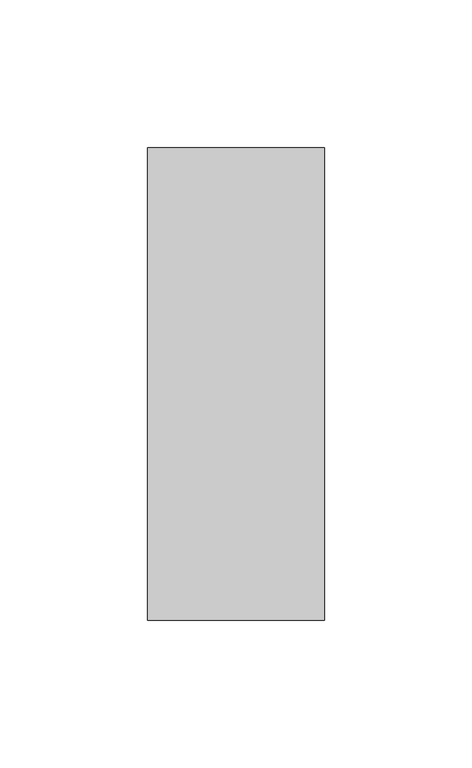
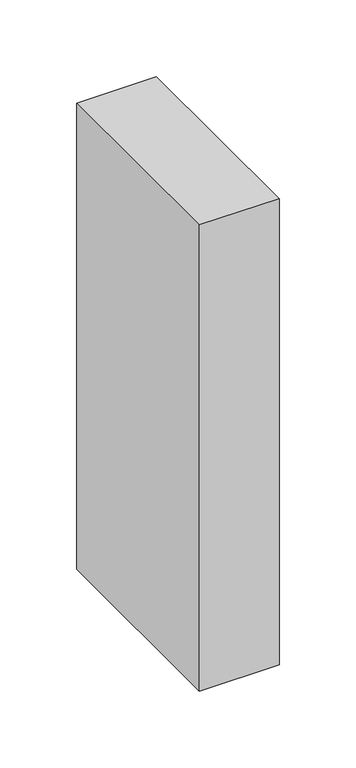
"""IFC4 building model written with IfcOpenShell, lengths in millimetres: column geometry, Madeira de lei-Coluna : Pontalete 6X16cm."""

import ifcopenshell
import ifcopenshell.guid

model = None  # the IFC model being written
_history = None  # IfcOwnerHistory: only IFC2X3 demands one
_inside = {}  # id of a spatial element -> (the spatial element, [elements in it])
_under = {}  # id of a project, library or spatial element -> (it, [spatial elements below it])
_declared = {}  # id of a project -> (the project, [libraries it declares])
_typed = {}  # id of a type object -> (the type object, [elements of that type])
_made_of = {}  # id of a material, layer set ... -> (it, [elements and type objects made of it])


def new_model(schema):
    """Start an empty IFC model of exactly this schema.

    Asked for "IFC4X3", IfcOpenShell would pick the latest addendum, in which some entities
    have other attributes; the version numbers below select the first issue.
    IFC2X3 requires an IfcOwnerHistory on every rooted entity: one is made here for all.
    """
    global model, _history
    if schema == "IFC4X3":
        model = ifcopenshell.file(schema_version=(4, 3, 0, 0))
    else:
        model = ifcopenshell.file(schema=schema)
    _inside.clear()
    _under.clear()
    _declared.clear()
    _typed.clear()
    _made_of.clear()
    _history = None
    if model.schema == "IFC2X3":
        org = make("IfcOrganization", Name="unknown")
        user = make(
            "IfcPersonAndOrganization",
            ThePerson=make("IfcPerson", FamilyName="unknown"),
            TheOrganization=org,
        )
        app = make(
            "IfcApplication",
            ApplicationDeveloper=org,
            Version="unknown",
            ApplicationFullName="unknown",
            ApplicationIdentifier="unknown",
        )
        _history = make(
            "IfcOwnerHistory",
            OwningUser=user,
            OwningApplication=app,
            ChangeAction="ADDED",
            CreationDate=0,
        )
    return model


def make(cls, **values):
    """One entity of the class cls with the attributes given. An attribute that is None is left unset."""
    return model.create_entity(
        cls, **{name: value for name, value in values.items() if value is not None}
    )


def rooted(cls, **values):
    """An entity with a GlobalId (a new one), such as an element, a storey or a relation."""
    return make(cls, GlobalId=ifcopenshell.guid.new(), OwnerHistory=_history, **values)


def si_unit(unit_type, name, prefix=None):
    """IfcSIUnit, for example si_unit("LENGTHUNIT", "METRE", prefix="MILLI")."""
    return make("IfcSIUnit", UnitType=unit_type, Prefix=prefix, Name=name)


def assignment(units):
    """IfcUnitAssignment: the units of a project."""
    return None if units is None else make("IfcUnitAssignment", Units=units)


def point(xyz):
    """IfcCartesianPoint."""
    return None if xyz is None else make("IfcCartesianPoint", Coordinates=xyz)


def direction(xyz):
    """IfcDirection."""
    return None if xyz is None else make("IfcDirection", DirectionRatios=xyz)


def frame(location, z_axis=None, x_axis=None):
    """IfcAxis2Placement3D, a coordinate frame: its origin and axes. An axis left out is left unset."""
    return make(
        "IfcAxis2Placement3D",
        Location=point(location),
        Axis=direction(z_axis),
        RefDirection=direction(x_axis),
    )


def origin():
    """The frame at (0, 0, 0) with its axes left unset."""
    return frame((0.0, 0.0, 0.0))


def place(relative_to, where):
    """IfcLocalPlacement: puts the frame where relative to a parent placement (None: the world)."""
    return make(
        "IfcLocalPlacement", PlacementRelTo=relative_to, RelativePlacement=where
    )


def context(
    kind, dimensions, precision=None, world=None, true_north=None, identifier=None
):
    """IfcGeometricRepresentationContext, for example the 3D "Model" context."""
    return make(
        "IfcGeometricRepresentationContext",
        ContextIdentifier=identifier,
        ContextType=kind,
        CoordinateSpaceDimension=dimensions,
        Precision=precision,
        WorldCoordinateSystem=world,
        TrueNorth=true_north,
    )


def project(units=None, contexts=None):
    """IfcProject with its units and contexts."""
    return rooted(
        "IfcProject",
        Name="project",
        RepresentationContexts=contexts,
        UnitsInContext=assignment(units),
    )


def spatial(cls, under=None, at=None, **own):
    """A site, building, storey or space (cls), placed at a placement, below another one or the project."""
    s = rooted(cls, ObjectPlacement=at, **own)
    if under is not None:
        _under.setdefault(under.id(), (under, []))[1].append(s)
    return s


def polyline(points):
    """IfcPolyline through the points."""
    return make("IfcPolyline", Points=[point(p) for p in points])


def outline(outer, holes=None, kind="AREA"):
    """IfcArbitraryClosedProfileDef: a profile drawn as a closed curve; with holes, ...WithVoids."""
    if holes is None:
        return make("IfcArbitraryClosedProfileDef", ProfileType=kind, OuterCurve=outer)
    return make(
        "IfcArbitraryProfileDefWithVoids",
        ProfileType=kind,
        OuterCurve=outer,
        InnerCurves=holes,
    )


def extrude(swept, where, along, depth):
    """IfcExtrudedAreaSolid: the profile swept, set in the frame where, extruded along a direction by depth."""
    return make(
        "IfcExtrudedAreaSolid",
        SweptArea=swept,
        Position=where,
        ExtrudedDirection=direction(along),
        Depth=depth,
    )


def shape(context_of_items, identifier, shape_type, items):
    """IfcShapeRepresentation: the items that make up one representation, for example the "Body"."""
    return make(
        "IfcShapeRepresentation",
        ContextOfItems=context_of_items,
        RepresentationIdentifier=identifier,
        RepresentationType=shape_type,
        Items=items,
    )


def source(mapping_origin, context_of_items, identifier, shape_type, items):
    """IfcRepresentationMap: a shape defined once, which mapped items show again and again."""
    return make(
        "IfcRepresentationMap",
        MappingOrigin=mapping_origin,
        MappedRepresentation=shape(context_of_items, identifier, shape_type, items),
    )


def transform(
    local_origin,
    x_axis=None,
    y_axis=None,
    z_axis=None,
    scale=None,
    scale2=None,
    scale3=None,
    uniform=True,
):
    """IfcCartesianTransformationOperator3D, or its non-uniform kind. x_axis, y_axis, z_axis: its Axis1, 2, 3."""
    if uniform:
        return make(
            "IfcCartesianTransformationOperator3D",
            Axis1=direction(x_axis),
            Axis2=direction(y_axis),
            LocalOrigin=point(local_origin),
            Scale=scale,
            Axis3=direction(z_axis),
        )
    return make(
        "IfcCartesianTransformationOperator3DnonUniform",
        Axis1=direction(x_axis),
        Axis2=direction(y_axis),
        LocalOrigin=point(local_origin),
        Scale=scale,
        Axis3=direction(z_axis),
        Scale2=scale2,
        Scale3=scale3,
    )


def mapped(mapping_source, mapping_target):
    """IfcMappedItem: shows the shape of a source again, moved by a transform."""
    return make(
        "IfcMappedItem", MappingSource=mapping_source, MappingTarget=mapping_target
    )


def made_of(thing, what):
    """Note that an element or type object is made of a material, layer set ...; save() writes the relation."""
    if what is not None:
        _made_of.setdefault(what.id(), (what, []))[1].append(thing)
    return thing


def element(
    cls,
    number,
    at=None,
    inside=None,
    cuts=None,
    type_object=None,
    material=None,
    context=None,
    identifier="Body",
    shape_type=None,
    held_by="IfcProductDefinitionShape",
    body=None,
    shapes=None,
    **own,
):
    """One element of the class cls, such as IfcWall. Its Tag is "e" and its number.

    at: its placement. inside: the storey or other place that contains it. cuts: it is an
    opening in that element (IfcRelVoidsElement). A single representation is given by context,
    identifier, shape_type and body (its items); several are given by shapes. held_by: the class
    of the entity that holds the representations. save() writes the other relations.
    """
    e = rooted(cls, Tag="e%d" % number, ObjectPlacement=at, **own)
    if body is not None:
        shapes = [shape(context, identifier, shape_type, body)]
    if shapes is not None:
        e.Representation = make(held_by, Representations=shapes)
    if inside is not None:
        _inside.setdefault(inside.id(), (inside, []))[1].append(e)
    if cuts is not None:
        rooted(
            "IfcRelVoidsElement", RelatingBuildingElement=cuts, RelatedOpeningElement=e
        )
    if type_object is not None:
        _typed.setdefault(type_object.id(), (type_object, []))[1].append(e)
    return made_of(e, material)


def aggregate(whole, parts):
    """IfcRelAggregates: a whole, such as a stair, and the parts it consists of."""
    return rooted("IfcRelAggregates", RelatingObject=whole, RelatedObjects=parts)


def save(model, path):
    """Write the relations noted so far, then the file.

    IfcRelAggregates (storeys below a building ...), IfcRelContainedInSpatialStructure (elements
    in a storey), IfcRelDefinesByType, IfcRelAssociatesMaterial and IfcRelDeclares: one each for
    every whole, place, type object, material and project.
    """
    for whole, parts in _under.values():
        aggregate(whole, parts)
    for where, things in _inside.values():
        rooted(
            "IfcRelContainedInSpatialStructure",
            RelatedElements=things,
            RelatingStructure=where,
        )
    for kind, things in _typed.values():
        rooted("IfcRelDefinesByType", RelatedObjects=things, RelatingType=kind)
    for what, things in _made_of.values():
        rooted("IfcRelAssociatesMaterial", RelatedObjects=things, RelatingMaterial=what)
    for by, libraries in _declared.values():
        rooted("IfcRelDeclares", RelatingContext=by, RelatedDefinitions=libraries)
    model.write(path)


def column_910cb117(model_context):
    return source(origin(), model_context, "Body", "SweptSolid", [
        extrude(outline(polyline([(30.0, 80.0), (30.0, -80.0), (-30.0, -80.0), (-30.0, 80.0), (30.0, 80.0)])), frame((0.0, 0.0, 6710.0), z_axis=(0.0, 0.0, 1.0), x_axis=(1.0, 0.0, 0.0)), (0.0, 0.0, 1.0), 371.3),
    ])


if __name__ == "__main__":
    model = new_model("IFC4")
    model_context = context("Model", 3, world=origin())
    ifc_project = project(units=[si_unit("LENGTHUNIT", "METRE", prefix="MILLI")], contexts=[model_context])
    site = spatial("IfcSite", under=ifc_project)
    building = spatial("IfcBuilding", under=site)
    placement = place(None, origin())
    column_shape = column_910cb117(model_context)
    element("IfcColumn", 1, ObjectType="Madeira de lei-Coluna : Pontalete 6X16cm", at=placement, inside=building, context=model_context, shape_type="MappedRepresentation", body=[
        mapped(column_shape, transform((0.0, 0.0, 0.0), x_axis=(1.0, 0.0, 0.0), y_axis=(0.0, 1.0, 0.0), z_axis=(0.0, 0.0, 1.0))),
    ])
    save(model, "model.ifc")

# Revit data of these elements
# Type "Madeira de lei-Coluna : Pontalete 6X16cm"
#   A = 0.01952 m²
#   b = 0.06 m
#   d = 0.16 m
#   Structural Material [instance default] = none
#   Assembly Code = ""
# Element 1 (IfcColumn, "Madeira de lei-Coluna : Pontalete 6X16cm")
#   Structural Material = .MADEIRAMENTO
#   Materials on its faces: ".MADEIRAMENTO"
# Materials
#   ".MADEIRAMENTO": class ".CC_MADEIRAS", colour RGB 212 179 113, transparency 0, Cost = 0
